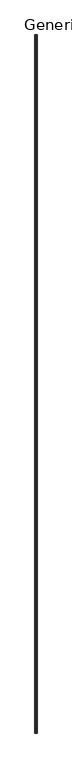
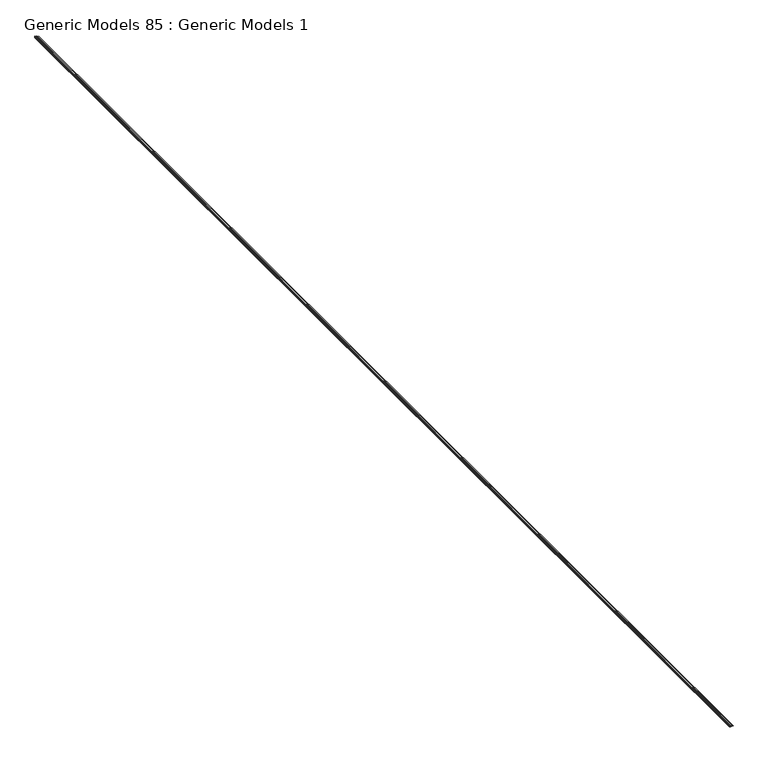
"""IFC4 building model written with IfcOpenShell, lengths in millimetres: proxy geometry, Generic Models 85 : Generic Models 1."""

import ifcopenshell
import ifcopenshell.guid

model = None  # the IFC model being written
_history = None  # IfcOwnerHistory: only IFC2X3 demands one
_inside = {}  # id of a spatial element -> (the spatial element, [elements in it])
_under = {}  # id of a project, library or spatial element -> (it, [spatial elements below it])
_declared = {}  # id of a project -> (the project, [libraries it declares])
_typed = {}  # id of a type object -> (the type object, [elements of that type])
_made_of = {}  # id of a material, layer set ... -> (it, [elements and type objects made of it])


def new_model(schema):
    """Start an empty IFC model of exactly this schema.

    Asked for "IFC4X3", IfcOpenShell would pick the latest addendum, in which some entities
    have other attributes; the version numbers below select the first issue.
    IFC2X3 requires an IfcOwnerHistory on every rooted entity: one is made here for all.
    """
    global model, _history
    if schema == "IFC4X3":
        model = ifcopenshell.file(schema_version=(4, 3, 0, 0))
    else:
        model = ifcopenshell.file(schema=schema)
    _inside.clear()
    _under.clear()
    _declared.clear()
    _typed.clear()
    _made_of.clear()
    _history = None
    if model.schema == "IFC2X3":
        org = make("IfcOrganization", Name="unknown")
        user = make(
            "IfcPersonAndOrganization",
            ThePerson=make("IfcPerson", FamilyName="unknown"),
            TheOrganization=org,
        )
        app = make(
            "IfcApplication",
            ApplicationDeveloper=org,
            Version="unknown",
            ApplicationFullName="unknown",
            ApplicationIdentifier="unknown",
        )
        _history = make(
            "IfcOwnerHistory",
            OwningUser=user,
            OwningApplication=app,
            ChangeAction="ADDED",
            CreationDate=0,
        )
    return model


def make(cls, **values):
    """One entity of the class cls with the attributes given. An attribute that is None is left unset."""
    return model.create_entity(
        cls, **{name: value for name, value in values.items() if value is not None}
    )


def rooted(cls, **values):
    """An entity with a GlobalId (a new one), such as an element, a storey or a relation."""
    return make(cls, GlobalId=ifcopenshell.guid.new(), OwnerHistory=_history, **values)


def si_unit(unit_type, name, prefix=None):
    """IfcSIUnit, for example si_unit("LENGTHUNIT", "METRE", prefix="MILLI")."""
    return make("IfcSIUnit", UnitType=unit_type, Prefix=prefix, Name=name)


def assignment(units):
    """IfcUnitAssignment: the units of a project."""
    return None if units is None else make("IfcUnitAssignment", Units=units)


def point(xyz):
    """IfcCartesianPoint."""
    return None if xyz is None else make("IfcCartesianPoint", Coordinates=xyz)


def direction(xyz):
    """IfcDirection."""
    return None if xyz is None else make("IfcDirection", DirectionRatios=xyz)


def frame(location, z_axis=None, x_axis=None):
    """IfcAxis2Placement3D, a coordinate frame: its origin and axes. An axis left out is left unset."""
    return make(
        "IfcAxis2Placement3D",
        Location=point(location),
        Axis=direction(z_axis),
        RefDirection=direction(x_axis),
    )


def origin():
    """The frame at (0, 0, 0) with its axes left unset."""
    return frame((0.0, 0.0, 0.0))


def place(relative_to, where):
    """IfcLocalPlacement: puts the frame where relative to a parent placement (None: the world)."""
    return make(
        "IfcLocalPlacement", PlacementRelTo=relative_to, RelativePlacement=where
    )


def context(
    kind, dimensions, precision=None, world=None, true_north=None, identifier=None
):
    """IfcGeometricRepresentationContext, for example the 3D "Model" context."""
    return make(
        "IfcGeometricRepresentationContext",
        ContextIdentifier=identifier,
        ContextType=kind,
        CoordinateSpaceDimension=dimensions,
        Precision=precision,
        WorldCoordinateSystem=world,
        TrueNorth=true_north,
    )


def project(units=None, contexts=None):
    """IfcProject with its units and contexts."""
    return rooted(
        "IfcProject",
        Name="project",
        RepresentationContexts=contexts,
        UnitsInContext=assignment(units),
    )


def spatial(cls, under=None, at=None, **own):
    """A site, building, storey or space (cls), placed at a placement, below another one or the project."""
    s = rooted(cls, ObjectPlacement=at, **own)
    if under is not None:
        _under.setdefault(under.id(), (under, []))[1].append(s)
    return s


def polyline(points):
    """IfcPolyline through the points."""
    return make("IfcPolyline", Points=[point(p) for p in points])


def outline(outer, holes=None, kind="AREA"):
    """IfcArbitraryClosedProfileDef: a profile drawn as a closed curve; with holes, ...WithVoids."""
    if holes is None:
        return make("IfcArbitraryClosedProfileDef", ProfileType=kind, OuterCurve=outer)
    return make(
        "IfcArbitraryProfileDefWithVoids",
        ProfileType=kind,
        OuterCurve=outer,
        InnerCurves=holes,
    )


def extrude(swept, where, along, depth):
    """IfcExtrudedAreaSolid: the profile swept, set in the frame where, extruded along a direction by depth."""
    return make(
        "IfcExtrudedAreaSolid",
        SweptArea=swept,
        Position=where,
        ExtrudedDirection=direction(along),
        Depth=depth,
    )


def shape(context_of_items, identifier, shape_type, items):
    """IfcShapeRepresentation: the items that make up one representation, for example the "Body"."""
    return make(
        "IfcShapeRepresentation",
        ContextOfItems=context_of_items,
        RepresentationIdentifier=identifier,
        RepresentationType=shape_type,
        Items=items,
    )


def source(mapping_origin, context_of_items, identifier, shape_type, items):
    """IfcRepresentationMap: a shape defined once, which mapped items show again and again."""
    return make(
        "IfcRepresentationMap",
        MappingOrigin=mapping_origin,
        MappedRepresentation=shape(context_of_items, identifier, shape_type, items),
    )


def transform(
    local_origin,
    x_axis=None,
    y_axis=None,
    z_axis=None,
    scale=None,
    scale2=None,
    scale3=None,
    uniform=True,
):
    """IfcCartesianTransformationOperator3D, or its non-uniform kind. x_axis, y_axis, z_axis: its Axis1, 2, 3."""
    if uniform:
        return make(
            "IfcCartesianTransformationOperator3D",
            Axis1=direction(x_axis),
            Axis2=direction(y_axis),
            LocalOrigin=point(local_origin),
            Scale=scale,
            Axis3=direction(z_axis),
        )
    return make(
        "IfcCartesianTransformationOperator3DnonUniform",
        Axis1=direction(x_axis),
        Axis2=direction(y_axis),
        LocalOrigin=point(local_origin),
        Scale=scale,
        Axis3=direction(z_axis),
        Scale2=scale2,
        Scale3=scale3,
    )


def mapped(mapping_source, mapping_target):
    """IfcMappedItem: shows the shape of a source again, moved by a transform."""
    return make(
        "IfcMappedItem", MappingSource=mapping_source, MappingTarget=mapping_target
    )


def made_of(thing, what):
    """Note that an element or type object is made of a material, layer set ...; save() writes the relation."""
    if what is not None:
        _made_of.setdefault(what.id(), (what, []))[1].append(thing)
    return thing


def element(
    cls,
    number,
    at=None,
    inside=None,
    cuts=None,
    type_object=None,
    material=None,
    context=None,
    identifier="Body",
    shape_type=None,
    held_by="IfcProductDefinitionShape",
    body=None,
    shapes=None,
    **own,
):
    """One element of the class cls, such as IfcWall. Its Tag is "e" and its number.

    at: its placement. inside: the storey or other place that contains it. cuts: it is an
    opening in that element (IfcRelVoidsElement). A single representation is given by context,
    identifier, shape_type and body (its items); several are given by shapes. held_by: the class
    of the entity that holds the representations. save() writes the other relations.
    """
    e = rooted(cls, Tag="e%d" % number, ObjectPlacement=at, **own)
    if body is not None:
        shapes = [shape(context, identifier, shape_type, body)]
    if shapes is not None:
        e.Representation = make(held_by, Representations=shapes)
    if inside is not None:
        _inside.setdefault(inside.id(), (inside, []))[1].append(e)
    if cuts is not None:
        rooted(
            "IfcRelVoidsElement", RelatingBuildingElement=cuts, RelatedOpeningElement=e
        )
    if type_object is not None:
        _typed.setdefault(type_object.id(), (type_object, []))[1].append(e)
    return made_of(e, material)


def aggregate(whole, parts):
    """IfcRelAggregates: a whole, such as a stair, and the parts it consists of."""
    return rooted("IfcRelAggregates", RelatingObject=whole, RelatedObjects=parts)


def save(model, path):
    """Write the relations noted so far, then the file.

    IfcRelAggregates (storeys below a building ...), IfcRelContainedInSpatialStructure (elements
    in a storey), IfcRelDefinesByType, IfcRelAssociatesMaterial and IfcRelDeclares: one each for
    every whole, place, type object, material and project.
    """
    for whole, parts in _under.values():
        aggregate(whole, parts)
    for where, things in _inside.values():
        rooted(
            "IfcRelContainedInSpatialStructure",
            RelatedElements=things,
            RelatingStructure=where,
        )
    for kind, things in _typed.values():
        rooted("IfcRelDefinesByType", RelatedObjects=things, RelatingType=kind)
    for what, things in _made_of.values():
        rooted("IfcRelAssociatesMaterial", RelatedObjects=things, RelatingMaterial=what)
    for by, libraries in _declared.values():
        rooted("IfcRelDeclares", RelatingContext=by, RelatedDefinitions=libraries)
    model.write(path)


def generic_models_85_generic_models_1_6d19cfd5(model_context):
    return source(origin(), model_context, "Body", "SweptSolid", [
        extrude(outline(polyline([(142822.070303, -9483.4874704), (142824.280103, -9483.4874704), (142824.280103, -9482.6286296), (142844.5946817, -9482.6286296), (142844.5946817, -9483.8986296), (142825.550103, -9483.8986296), (142825.550103, -9484.7574704), (142820.800303, -9484.7574704), (142820.800303, -9462.5324704), (142832.230303, -9462.5324704), (142832.230303, -9449.8324704), (142820.800303, -9449.8324704), (142820.800303, -9426.1192865), (142822.070303, -9426.1192865), (142822.070303, -9448.5624704), (142833.500303, -9448.5624704), (142833.500303, -9463.8024704), (142822.070303, -9463.8024704), (142822.070303, -9483.4874704)])), frame((0.0, -7068.1230338, 0.0), z_axis=(0.0, 1.0, 0.0), x_axis=(0.0, 0.0, 1.0)), (0.0, 0.0, 1.0), 19050.0),
    ])


if __name__ == "__main__":
    model = new_model("IFC4")
    model_context = context("Model", 3, world=origin())
    ifc_project = project(units=[si_unit("LENGTHUNIT", "METRE", prefix="MILLI")], contexts=[model_context])
    site = spatial("IfcSite", under=ifc_project)
    building = spatial("IfcBuilding", under=site)
    placement = place(None, origin())
    generic_models_85_generic_models_1_shape = generic_models_85_generic_models_1_6d19cfd5(model_context)
    element("IfcBuildingElementProxy", 1, Name="Generic Models 85 : Generic Models 1", ObjectType="Generic Models 85 : Generic Models 1", at=placement, inside=building, context=model_context, shape_type="MappedRepresentation", body=[
        mapped(generic_models_85_generic_models_1_shape, transform((0.0, 0.0, 0.0), x_axis=(1.0, 0.0, 0.0), y_axis=(0.0, 1.0, 0.0), z_axis=(0.0, 0.0, 1.0))),
    ])
    save(model, "model.ifc")

# Revit data of these elements
# Element 1 (IfcBuildingElementProxy, "Generic Models 85 : Generic Models 1")
#   Materials on its faces: "_16 GA. COPPER SOFFIT DRIP SCREED"
# Materials
#   "_16 GA. COPPER SOFFIT DRIP SCREED": class "Generic", colour RGB 253 192 103, transparency 0, Cost = 0
